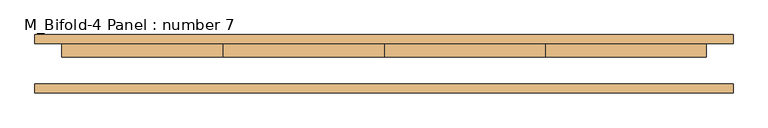
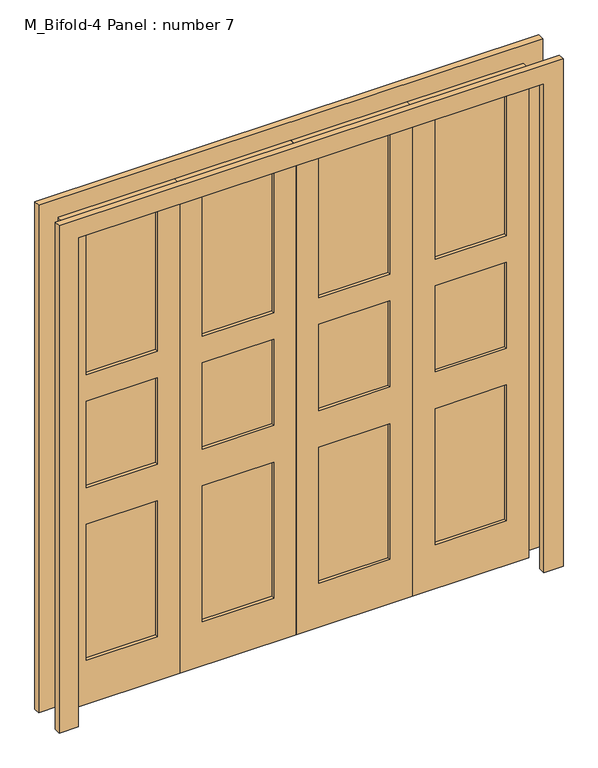
"""IFC4 building model written with IfcOpenShell, lengths in millimetres: door geometry, M_Bifold-4 Panel : number 7."""

from ifc_helpers import new_model, si_unit, frame, origin, place, context, project, spatial, polyline, outline, extrude, source, transform, mapped, element, save


def m_bifold_4_panel_number_7_e3611513(model_context):
    return source(origin(), model_context, "Body", "SweptSolid", [
        extrude(outline(polyline([(546.1, 44.45), (825.5, 44.45), (825.5, 31.75), (546.1, 31.75), (546.1, 44.45)])), frame((0.0, 0.0, 1370.1314325), z_axis=(0.0, 0.0, 1.0), x_axis=(1.0, 0.0, 0.0)), (0.0, 0.0, 1.0), 579.3185675),
        extrude(outline(polyline([(546.1, 44.45), (825.5, 44.45), (825.5, 31.75), (546.1, 31.75), (546.1, 44.45)])), frame((0.0, 0.0, 184.15), z_axis=(0.0, 0.0, 1.0), x_axis=(1.0, 0.0, 0.0)), (0.0, 0.0, 1.0), 565.15),
        extrude(outline(polyline([(88.6, 44.45), (368.3, 44.45), (368.3, 31.75), (88.6, 31.75), (88.6, 44.45)])), frame((0.0, 0.0, 1370.1314325), z_axis=(0.0, 0.0, 1.0), x_axis=(1.0, 0.0, 0.0)), (0.0, 0.0, 1.0), 579.3185675),
        extrude(outline(polyline([(88.9, 44.45), (368.3, 44.45), (368.3, 31.75), (88.9, 31.75), (88.9, 44.45)])), frame((0.0, 0.0, 184.15), z_axis=(0.0, 0.0, 1.0), x_axis=(1.0, 0.0, 0.0)), (0.0, 0.0, 1.0), 565.15),
        extrude(outline(polyline([(-368.3, 44.45), (-88.9, 44.45), (-88.9, 31.75), (-368.3, 31.75), (-368.3, 44.45)])), frame((0.0, 0.0, 184.15), z_axis=(0.0, 0.0, 1.0), x_axis=(1.0, 0.0, 0.0)), (0.0, 0.0, 1.0), 565.15),
        extrude(outline(polyline([(-368.9, 44.45), (-89.2, 44.45), (-89.2, 31.75), (-368.9, 31.75), (-368.9, 44.45)])), frame((0.0, 0.0, 1370.1314325), z_axis=(0.0, 0.0, 1.0), x_axis=(1.0, 0.0, 0.0)), (0.0, 0.0, 1.0), 579.3185675),
        extrude(outline(polyline([(-826.4, 44.45), (-546.7, 44.45), (-546.7, 31.75), (-826.4, 31.75), (-826.4, 44.45)])), frame((0.0, 0.0, 1370.1314325), z_axis=(0.0, 0.0, 1.0), x_axis=(1.0, 0.0, 0.0)), (0.0, 0.0, 1.0), 579.3185675),
        extrude(outline(polyline([(-825.8, 44.45), (-546.1, 44.45), (-546.1, 31.75), (-825.8, 31.75), (-825.8, 44.45)])), frame((0.0, 0.0, 184.15), z_axis=(0.0, 0.0, 1.0), x_axis=(1.0, 0.0, 0.0)), (0.0, 0.0, 1.0), 565.15),
        extrude(outline(polyline([(-368.9, 44.45), (-88.9, 44.45), (-88.9, 31.75), (-368.9, 31.75), (-368.9, 44.45)])), frame((0.0, 0.0, 901.1314325), z_axis=(0.0, 0.0, 1.0), x_axis=(1.0, 0.0, 0.0)), (0.0, 0.0, 1.0), 359.3185675),
        extrude(outline(polyline([(88.9, 44.45), (368.3, 44.45), (368.3, 31.75), (88.9, 31.75), (88.9, 44.45)])), frame((0.0, 0.0, 901.1314325), z_axis=(0.0, 0.0, 1.0), x_axis=(1.0, 0.0, 0.0)), (0.0, 0.0, 1.0), 359.3185675),
        extrude(outline(polyline([(546.1, 44.45), (825.5, 44.45), (825.5, 31.75), (546.1, 31.75), (546.1, 44.45)])), frame((0.0, 0.0, 901.1314325), z_axis=(0.0, 0.0, 1.0), x_axis=(1.0, 0.0, 0.0)), (0.0, 0.0, 1.0), 359.3185675),
        extrude(outline(polyline([(-826.4, 44.45), (-546.7, 44.45), (-546.7, 31.75), (-826.4, 31.75), (-826.4, 44.45)])), frame((0.0, 0.0, 901.1314325), z_axis=(0.0, 0.0, 1.0), x_axis=(1.0, 0.0, 0.0)), (0.0, 0.0, 1.0), 359.3185675),
        extrude(outline(polyline([(0.0, 990.4), (2108.0, 990.4), (2108.0, -990.4), (0.0, -990.4), (0.0, -914.4), (2032.0, -914.4), (2032.0, 914.4), (0.0, 914.4), (0.0, 990.4)])), frame((0.0, -82.55, 0.0), z_axis=(0.0, 1.0, 0.0), x_axis=(0.0, 0.0, 1.0)), (0.0, 0.0, 1.0), 25.4),
        extrude(outline(polyline([(0.0, 990.4), (2108.0, 990.4), (2108.0, -990.4), (0.0, -990.4), (0.0, -914.4), (2032.0, -914.4), (2032.0, 914.4), (0.0, 914.4), (0.0, 990.4)])), frame((0.0, 57.15, 0.0), z_axis=(0.0, 1.0, 0.0), x_axis=(0.0, 0.0, 1.0)), (0.0, 0.0, 1.0), 25.4),
        extrude(outline(polyline([(0.0, -914.4), (0.0, -457.2), (2032.0, -457.2), (2032.0, -914.4), (0.0, -914.4)]), holes=[polyline([(1949.45, -825.5), (1949.45, -546.1), (1370.1314325, -546.1), (1370.1314325, -825.5), (1949.45, -825.5)]), polyline([(749.3, -825.5), (749.3, -546.1), (184.15, -546.1), (184.15, -825.5), (749.3, -825.5)]), polyline([(1260.45, -825.5), (1260.45, -546.1), (901.1314325, -546.1), (901.1314325, -825.5), (1260.45, -825.5)])]), frame((0.0, 19.05, 0.0), z_axis=(0.0, 1.0, 0.0), x_axis=(0.0, 0.0, 1.0)), (0.0, 0.0, 1.0), 38.1),
        extrude(outline(polyline([(0.0, -457.2), (0.0, 0.0), (2032.0, 0.0), (2032.0, -457.2), (0.0, -457.2)]), holes=[polyline([(1949.45, -368.3), (1949.45, -88.9), (1370.1314325, -88.9), (1370.1314325, -368.3), (1949.45, -368.3)]), polyline([(749.3, -368.3), (749.3, -88.9), (184.15, -88.9), (184.15, -368.3), (749.3, -368.3)]), polyline([(1260.45, -368.3), (1260.45, -88.9), (901.1314325, -88.9), (901.1314325, -368.3), (1260.45, -368.3)])]), frame((0.0, 19.05, 0.0), z_axis=(0.0, 1.0, 0.0), x_axis=(0.0, 0.0, 1.0)), (0.0, 0.0, 1.0), 38.1),
        extrude(outline(polyline([(0.0, 0.0), (0.0, 457.2), (2032.0, 457.2), (2032.0, 0.0), (0.0, 0.0)]), holes=[polyline([(1949.45, 88.9), (1949.45, 368.3), (1370.1314325, 368.3), (1370.1314325, 88.9), (1949.45, 88.9)]), polyline([(749.3, 88.9), (749.3, 368.3), (184.15, 368.3), (184.15, 88.9), (749.3, 88.9)]), polyline([(1260.45, 88.9), (1260.45, 368.3), (901.1314325, 368.3), (901.1314325, 88.9), (1260.45, 88.9)])]), frame((0.0, 19.05, 0.0), z_axis=(0.0, 1.0, 0.0), x_axis=(0.0, 0.0, 1.0)), (0.0, 0.0, 1.0), 38.1),
        extrude(outline(polyline([(0.0, 457.2), (0.0, 914.4), (2032.0, 914.4), (2032.0, 457.2), (0.0, 457.2)]), holes=[polyline([(1949.45, 546.1), (1949.45, 825.5), (1370.1314325, 825.5), (1370.1314325, 546.1), (1949.45, 546.1)]), polyline([(749.3, 546.1), (749.3, 825.5), (184.15, 825.5), (184.15, 546.1), (749.3, 546.1)]), polyline([(1260.45, 546.1), (1260.45, 825.5), (901.1314325, 825.5), (901.1314325, 546.1), (1260.45, 546.1)])]), frame((0.0, 19.05, 0.0), z_axis=(0.0, 1.0, 0.0), x_axis=(0.0, 0.0, 1.0)), (0.0, 0.0, 1.0), 38.1),
    ])


if __name__ == "__main__":
    model = new_model("IFC4")
    model_context = context("Model", 3, world=origin())
    ifc_project = project(units=[si_unit("LENGTHUNIT", "METRE", prefix="MILLI")], contexts=[model_context])
    site = spatial("IfcSite", under=ifc_project)
    building = spatial("IfcBuilding", under=site)
    placement = place(None, origin())
    m_bifold_4_panel_number_7_shape = m_bifold_4_panel_number_7_e3611513(model_context)
    element("IfcDoor", 1, ObjectType="M_Bifold-4 Panel : number 7", at=placement, inside=building, context=model_context, shape_type="MappedRepresentation", body=[
        mapped(m_bifold_4_panel_number_7_shape, transform((0.0, 0.0, 0.0), x_axis=(1.0, 0.0, 0.0), y_axis=(0.0, 1.0, 0.0), z_axis=(0.0, 0.0, 1.0))),
    ])
    save(model, "model.ifc")

# Revit data of these elements
# Type "M_Bifold-4 Panel : number 7"
#   Type Mark = "89"
#   Analytic Construction = "<None>"
#   Thickness = 0' - 1 3/4"
#   Height = 6' - 8"
#   Trim Width = 0' - 2.99213"
#   Width = 6' - 0"
#   Define Thermal Properties by = 1
#   Door Material = Door - Panel
#   Frame Material = Door - Frame
#   Function = (empty or 0)
#   Assembly Code = ""
#   Description = (empty or 0)
#   Wall Closure = (empty or 0)
# Element 1 (IfcDoor, "M_Bifold-4 Panel : number 7")
#   Materials on its faces: "Door - Panel", "Door - Frame"
# Materials
#   "Door - Panel": class "Wood", colour RGB 210 159 95, transparency 0, Keynote = "L20", Cost = 0
#   "Door - Frame": class "Miscellaneous", colour RGB 118 70 51, transparency 0
